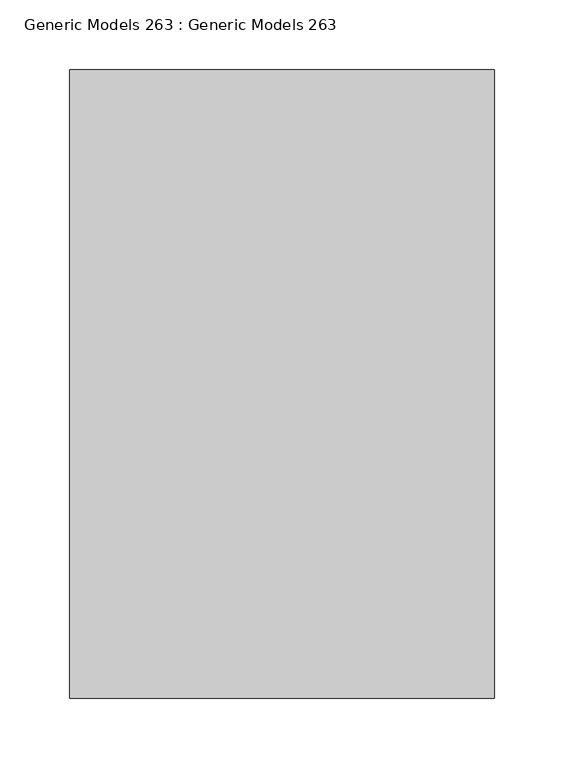
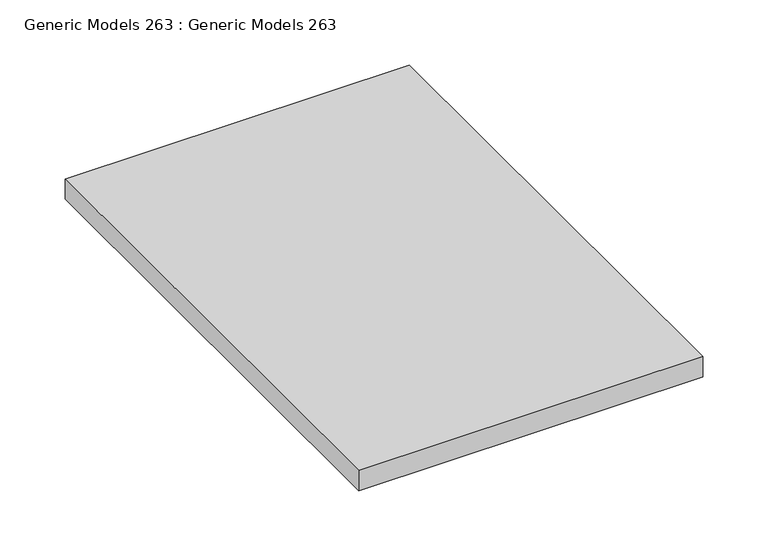
"""IFC4 building model written with IfcOpenShell, lengths in millimetres: proxy geometry, Generic Models 263 : Generic Models 263."""

import ifcopenshell
import ifcopenshell.guid

model = None  # the IFC model being written
_history = None  # IfcOwnerHistory: only IFC2X3 demands one
_inside = {}  # id of a spatial element -> (the spatial element, [elements in it])
_under = {}  # id of a project, library or spatial element -> (it, [spatial elements below it])
_declared = {}  # id of a project -> (the project, [libraries it declares])
_typed = {}  # id of a type object -> (the type object, [elements of that type])
_made_of = {}  # id of a material, layer set ... -> (it, [elements and type objects made of it])


def new_model(schema):
    """Start an empty IFC model of exactly this schema.

    Asked for "IFC4X3", IfcOpenShell would pick the latest addendum, in which some entities
    have other attributes; the version numbers below select the first issue.
    IFC2X3 requires an IfcOwnerHistory on every rooted entity: one is made here for all.
    """
    global model, _history
    if schema == "IFC4X3":
        model = ifcopenshell.file(schema_version=(4, 3, 0, 0))
    else:
        model = ifcopenshell.file(schema=schema)
    _inside.clear()
    _under.clear()
    _declared.clear()
    _typed.clear()
    _made_of.clear()
    _history = None
    if model.schema == "IFC2X3":
        org = make("IfcOrganization", Name="unknown")
        user = make(
            "IfcPersonAndOrganization",
            ThePerson=make("IfcPerson", FamilyName="unknown"),
            TheOrganization=org,
        )
        app = make(
            "IfcApplication",
            ApplicationDeveloper=org,
            Version="unknown",
            ApplicationFullName="unknown",
            ApplicationIdentifier="unknown",
        )
        _history = make(
            "IfcOwnerHistory",
            OwningUser=user,
            OwningApplication=app,
            ChangeAction="ADDED",
            CreationDate=0,
        )
    return model


def make(cls, **values):
    """One entity of the class cls with the attributes given. An attribute that is None is left unset."""
    return model.create_entity(
        cls, **{name: value for name, value in values.items() if value is not None}
    )


def rooted(cls, **values):
    """An entity with a GlobalId (a new one), such as an element, a storey or a relation."""
    return make(cls, GlobalId=ifcopenshell.guid.new(), OwnerHistory=_history, **values)


def si_unit(unit_type, name, prefix=None):
    """IfcSIUnit, for example si_unit("LENGTHUNIT", "METRE", prefix="MILLI")."""
    return make("IfcSIUnit", UnitType=unit_type, Prefix=prefix, Name=name)


def assignment(units):
    """IfcUnitAssignment: the units of a project."""
    return None if units is None else make("IfcUnitAssignment", Units=units)


def point(xyz):
    """IfcCartesianPoint."""
    return None if xyz is None else make("IfcCartesianPoint", Coordinates=xyz)


def direction(xyz):
    """IfcDirection."""
    return None if xyz is None else make("IfcDirection", DirectionRatios=xyz)


def frame(location, z_axis=None, x_axis=None):
    """IfcAxis2Placement3D, a coordinate frame: its origin and axes. An axis left out is left unset."""
    return make(
        "IfcAxis2Placement3D",
        Location=point(location),
        Axis=direction(z_axis),
        RefDirection=direction(x_axis),
    )


def origin():
    """The frame at (0, 0, 0) with its axes left unset."""
    return frame((0.0, 0.0, 0.0))


def place(relative_to, where):
    """IfcLocalPlacement: puts the frame where relative to a parent placement (None: the world)."""
    return make(
        "IfcLocalPlacement", PlacementRelTo=relative_to, RelativePlacement=where
    )


def context(
    kind, dimensions, precision=None, world=None, true_north=None, identifier=None
):
    """IfcGeometricRepresentationContext, for example the 3D "Model" context."""
    return make(
        "IfcGeometricRepresentationContext",
        ContextIdentifier=identifier,
        ContextType=kind,
        CoordinateSpaceDimension=dimensions,
        Precision=precision,
        WorldCoordinateSystem=world,
        TrueNorth=true_north,
    )


def project(units=None, contexts=None):
    """IfcProject with its units and contexts."""
    return rooted(
        "IfcProject",
        Name="project",
        RepresentationContexts=contexts,
        UnitsInContext=assignment(units),
    )


def spatial(cls, under=None, at=None, **own):
    """A site, building, storey or space (cls), placed at a placement, below another one or the project."""
    s = rooted(cls, ObjectPlacement=at, **own)
    if under is not None:
        _under.setdefault(under.id(), (under, []))[1].append(s)
    return s


def polyline(points):
    """IfcPolyline through the points."""
    return make("IfcPolyline", Points=[point(p) for p in points])


def outline(outer, holes=None, kind="AREA"):
    """IfcArbitraryClosedProfileDef: a profile drawn as a closed curve; with holes, ...WithVoids."""
    if holes is None:
        return make("IfcArbitraryClosedProfileDef", ProfileType=kind, OuterCurve=outer)
    return make(
        "IfcArbitraryProfileDefWithVoids",
        ProfileType=kind,
        OuterCurve=outer,
        InnerCurves=holes,
    )


def extrude(swept, where, along, depth):
    """IfcExtrudedAreaSolid: the profile swept, set in the frame where, extruded along a direction by depth."""
    return make(
        "IfcExtrudedAreaSolid",
        SweptArea=swept,
        Position=where,
        ExtrudedDirection=direction(along),
        Depth=depth,
    )


def shape(context_of_items, identifier, shape_type, items):
    """IfcShapeRepresentation: the items that make up one representation, for example the "Body"."""
    return make(
        "IfcShapeRepresentation",
        ContextOfItems=context_of_items,
        RepresentationIdentifier=identifier,
        RepresentationType=shape_type,
        Items=items,
    )


def source(mapping_origin, context_of_items, identifier, shape_type, items):
    """IfcRepresentationMap: a shape defined once, which mapped items show again and again."""
    return make(
        "IfcRepresentationMap",
        MappingOrigin=mapping_origin,
        MappedRepresentation=shape(context_of_items, identifier, shape_type, items),
    )


def transform(
    local_origin,
    x_axis=None,
    y_axis=None,
    z_axis=None,
    scale=None,
    scale2=None,
    scale3=None,
    uniform=True,
):
    """IfcCartesianTransformationOperator3D, or its non-uniform kind. x_axis, y_axis, z_axis: its Axis1, 2, 3."""
    if uniform:
        return make(
            "IfcCartesianTransformationOperator3D",
            Axis1=direction(x_axis),
            Axis2=direction(y_axis),
            LocalOrigin=point(local_origin),
            Scale=scale,
            Axis3=direction(z_axis),
        )
    return make(
        "IfcCartesianTransformationOperator3DnonUniform",
        Axis1=direction(x_axis),
        Axis2=direction(y_axis),
        LocalOrigin=point(local_origin),
        Scale=scale,
        Axis3=direction(z_axis),
        Scale2=scale2,
        Scale3=scale3,
    )


def mapped(mapping_source, mapping_target):
    """IfcMappedItem: shows the shape of a source again, moved by a transform."""
    return make(
        "IfcMappedItem", MappingSource=mapping_source, MappingTarget=mapping_target
    )


def made_of(thing, what):
    """Note that an element or type object is made of a material, layer set ...; save() writes the relation."""
    if what is not None:
        _made_of.setdefault(what.id(), (what, []))[1].append(thing)
    return thing


def element(
    cls,
    number,
    at=None,
    inside=None,
    cuts=None,
    type_object=None,
    material=None,
    context=None,
    identifier="Body",
    shape_type=None,
    held_by="IfcProductDefinitionShape",
    body=None,
    shapes=None,
    **own,
):
    """One element of the class cls, such as IfcWall. Its Tag is "e" and its number.

    at: its placement. inside: the storey or other place that contains it. cuts: it is an
    opening in that element (IfcRelVoidsElement). A single representation is given by context,
    identifier, shape_type and body (its items); several are given by shapes. held_by: the class
    of the entity that holds the representations. save() writes the other relations.
    """
    e = rooted(cls, Tag="e%d" % number, ObjectPlacement=at, **own)
    if body is not None:
        shapes = [shape(context, identifier, shape_type, body)]
    if shapes is not None:
        e.Representation = make(held_by, Representations=shapes)
    if inside is not None:
        _inside.setdefault(inside.id(), (inside, []))[1].append(e)
    if cuts is not None:
        rooted(
            "IfcRelVoidsElement", RelatingBuildingElement=cuts, RelatedOpeningElement=e
        )
    if type_object is not None:
        _typed.setdefault(type_object.id(), (type_object, []))[1].append(e)
    return made_of(e, material)


def aggregate(whole, parts):
    """IfcRelAggregates: a whole, such as a stair, and the parts it consists of."""
    return rooted("IfcRelAggregates", RelatingObject=whole, RelatedObjects=parts)


def save(model, path):
    """Write the relations noted so far, then the file.

    IfcRelAggregates (storeys below a building ...), IfcRelContainedInSpatialStructure (elements
    in a storey), IfcRelDefinesByType, IfcRelAssociatesMaterial and IfcRelDeclares: one each for
    every whole, place, type object, material and project.
    """
    for whole, parts in _under.values():
        aggregate(whole, parts)
    for where, things in _inside.values():
        rooted(
            "IfcRelContainedInSpatialStructure",
            RelatedElements=things,
            RelatingStructure=where,
        )
    for kind, things in _typed.values():
        rooted("IfcRelDefinesByType", RelatedObjects=things, RelatingType=kind)
    for what, things in _made_of.values():
        rooted("IfcRelAssociatesMaterial", RelatedObjects=things, RelatingMaterial=what)
    for by, libraries in _declared.values():
        rooted("IfcRelDeclares", RelatingContext=by, RelatedDefinitions=libraries)
    model.write(path)


def generic_models_263_generic_models_263_eb43eb0a(model_context):
    return source(origin(), model_context, "Body", "SweptSolid", [
        extrude(outline(polyline([(1389.5910488, 11321.4769662), (1389.5910488, 10870.6269662), (1084.7910488, 10870.6269662), (1084.7910488, 11321.4769662), (1389.5910488, 11321.4769662)])), frame((0.0, 0.0, 126840.996), z_axis=(0.0, 0.0, 1.0), x_axis=(1.0, 0.0, 0.0)), (0.0, 0.0, 1.0), 19.05),
    ])


if __name__ == "__main__":
    model = new_model("IFC4")
    model_context = context("Model", 3, world=origin())
    ifc_project = project(units=[si_unit("LENGTHUNIT", "METRE", prefix="MILLI")], contexts=[model_context])
    site = spatial("IfcSite", under=ifc_project)
    building = spatial("IfcBuilding", under=site)
    placement = place(None, origin())
    generic_models_263_generic_models_263_shape = generic_models_263_generic_models_263_eb43eb0a(model_context)
    element("IfcBuildingElementProxy", 1, Name="Generic Models 263 : Generic Models 263", ObjectType="Generic Models 263 : Generic Models 263", at=placement, inside=building, context=model_context, shape_type="MappedRepresentation", body=[
        mapped(generic_models_263_generic_models_263_shape, transform((0.0, 0.0, 0.0), x_axis=(1.0, 0.0, 0.0), y_axis=(0.0, 1.0, 0.0), z_axis=(0.0, 0.0, 1.0))),
    ])
    save(model, "model.ifc")

# Revit data of these elements
# Element 1 (IfcBuildingElementProxy, "Generic Models 263 : Generic Models 263")
#   Materials on its faces: "_WOOD FLOORING (SPEC T.B.D.)"
# Materials
#   "_WOOD FLOORING (SPEC T.B.D.)": class "Generic", colour RGB 177 130 114, transparency 0, Cost = 0
